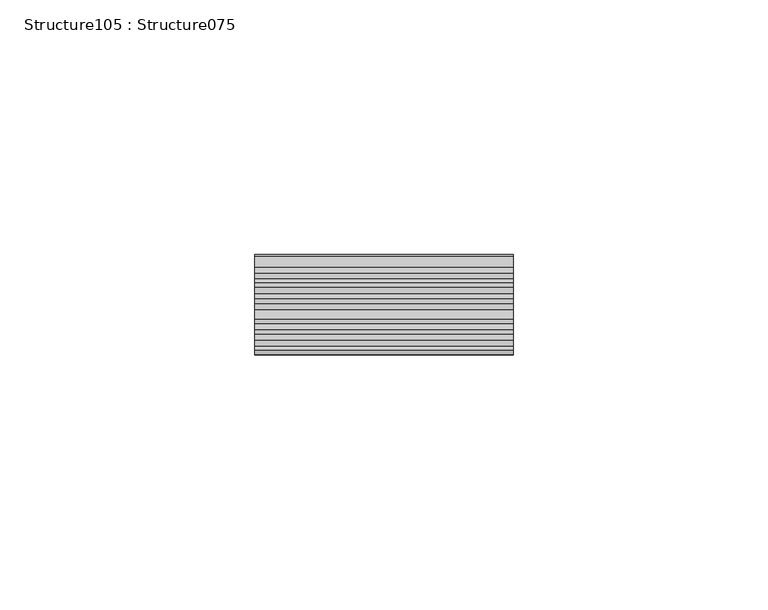
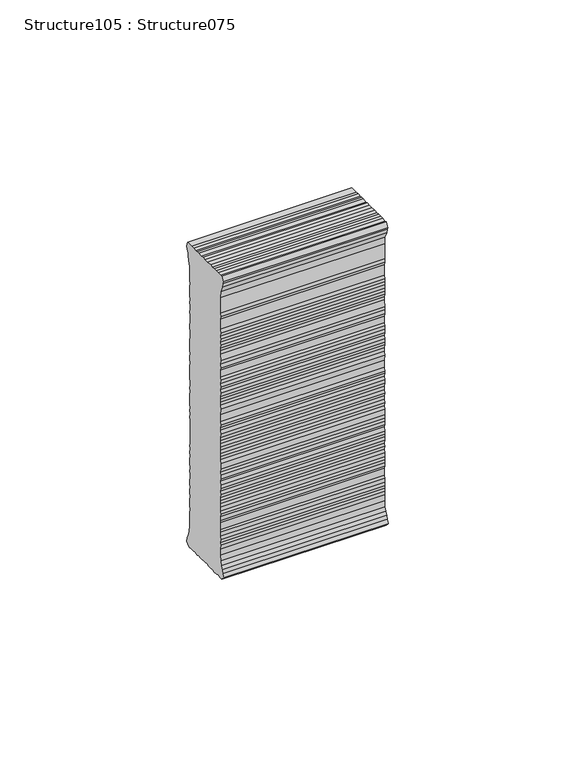
"""IFC4 building model written with IfcOpenShell, lengths in millimetres: proxy geometry, Structure105 : Structure075."""

from ifc_helpers import new_model, si_unit, frame, origin, place, context, project, spatial, polyline, outline, extrude, source, transform, mapped, element, save


def structure105_structure075_dffd82cc(model_context):
    return source(origin(), model_context, "Body", "SweptSolid", [
        extrude(outline(polyline([(1.8233335, 0.0), (3.1470297, 0.293028), (4.2244865, 0.737662), (5.4061289, 0.9114746), (6.4793271, 1.3564168), (7.453505, 0.3744049), (7.3876839, -0.5348157), (7.0413299, -1.6823692), (7.2469213, -2.4792419), (7.1626024, -3.6439812), (6.9587855, -4.6705706), (7.0218141, -5.5887623), (6.8180229, -6.6149967), (6.6191448, -7.5142283), (6.677363, -8.5580034), (6.5082886, -10.8935151), (6.3003415, -11.9180218), (6.5059586, -12.7145395), (6.1595789, -13.8624479), (6.2363462, -14.6499946), (6.1423932, -15.9478166), (6.1963785, -16.9909285), (6.0112391, -17.759515), (5.0532803, -18.342299), (3.7708431, -18.1196038), (2.7725399, -17.5250563), (1.8899032, -17.0723054), (1.0114786, -16.6155787), (-1.0399, -16.2077185), (-2.0754605, -16.1327513), (-3.1246312, -16.1866547), (-5.1943325, -16.036823), (-6.3503054, -15.693427), (-7.5226219, -15.7384156), (-8.43871, -15.8019532), (-9.3454464, -15.736312), (-10.6227907, -15.3841295), (-11.6774093, -15.5674945), (-12.7168735, -15.4922447), (-13.5992284, -15.1686566), (-14.5213496, -15.2317576), (-15.6843145, -15.1475672), (-16.7108781, -14.9433954), (-17.7503424, -14.8681455), (-18.7938349, -14.9224601), (-19.9492226, -14.7089623), (-21.0077449, -14.8920446), (-21.9144813, -14.8264034), (-22.8118661, -14.6315832), (-23.8366554, -14.4275398), (-24.8819223, -14.4817259), (-26.0451176, -14.2676629), (-26.9573019, -14.3314832), (-28.1165932, -14.1177028), (-35.504632, -13.5828614), (-36.2915412, -13.6557508), (-37.5800115, -13.4326187), (-38.6231492, -13.4869589), (-39.3938393, -13.3013105), (-40.5661558, -13.3462991), (-41.4822438, -13.4098367), (-42.5127113, -13.2053823), (-43.6850278, -13.2503708), (-44.8310639, -12.9076942), (-45.7510557, -12.9709493), (-46.904669, -12.7575799), (-47.9441332, -12.6823301), (-48.9987517, -12.8656951), (-50.9453073, -12.7247783), (-51.8391432, -12.5302151), (-53.1348358, -12.4364162), (-54.0325755, -12.2415703), (-55.2105702, -12.2861478), (-56.2447111, -12.2112834), (-57.1420959, -12.0164631), (-58.057829, -12.0800265), (-60.395825, -11.9107723), (-61.434704, -11.9654207), (-62.4561747, -11.6317617), (-64.2753257, -11.5000681), (-65.4479971, -11.545031), (-66.358407, -11.6089797), (-67.514025, -11.2656093), (-69.5837263, -11.1157777), (-70.5095209, -11.3084686), (-71.7865103, -10.9563118), (-72.8220707, -10.8813446), (-73.6093348, -10.9542083), (-74.7633029, -10.7408132), (-75.814248, -10.7945883), (-76.7303361, -10.8581259), (-78.9327652, -10.6986857), (-79.8207983, -10.3746866), (-80.9987931, -10.4192641), (-85.2712784, -10.1099666), (-87.1286228, -10.4960018), (-88.4487235, -10.7935711), (-89.368916, -10.8546711), (-90.3000349, -11.180043), (-91.3524984, -11.3632072), (-92.6260665, -10.8800153), (-92.4666006, -8.6772313), (-92.5113322, -7.501366), (-92.307032, -6.4730278), (-92.3799983, -5.6871834), (-92.3142543, -4.7790274), (-91.9643553, -3.5036582), (-92.1549168, -2.5780178), (-91.950591, -1.5493248), (-91.7392225, -0.393783), (-91.86404, 1.4400135), (-91.5421703, 2.3282008), (-91.7139001, 3.5139734), (-91.5191057, 4.4110033), (-91.5637858, 5.5875785), (-91.2230844, 6.735898), (-91.4229975, 7.5323595), (-89.9359318, 8.2045553), (-89.1900807, 7.7595664), (-87.9038939, 7.5344593), (-85.9090056, 6.3511965), (-83.842777, 6.0696199), (-78.9197837, 5.7132303), (-77.74128, 5.7599113), (-76.8537302, 5.4341636), (-73.4823032, 5.1900963), (-72.4272012, 5.3752099), (-71.4032759, 5.1690886), (-70.4866788, 5.2347299), (-69.3275415, 5.0188203), (-68.4109444, 5.0844615), (-67.3845349, 4.8781604), (-66.4867694, 4.6836695), (-65.4473053, 4.6084197), (-63.3587722, 4.7187202), (-62.199635, 4.5028106), (-61.0268094, 4.5499027), (-60.1335814, 4.2237439), (-57.9364757, 4.0646891), (-57.137957, 4.2683775), (-55.8517702, 4.0432704), (-54.8059941, 4.09956), (-53.9145406, 3.7735296), (-52.8597935, 3.9586689), (-51.7063344, 3.7431704), (-50.799598, 3.6775291), (-49.7726538, 3.4736865), (-48.7331896, 3.3984367), (-47.5457148, 3.5739675), (-45.7507187, 3.1825271), (-43.4191107, 3.0137353), (-42.3664931, 3.1990287), (-41.5959571, 3.011251), (-40.565464, 2.8071516), (-39.5128462, 2.992445), (-38.2305631, 2.7676205), (-37.20007, 2.563521), (-36.1641547, 2.4885281), (-35.1189134, 2.5423592), (-34.0887752, 2.3382854), (-33.0546342, 2.263421), (-32.0058441, 2.3169952), (-30.9792548, 2.1131783), (-29.9245077, 2.2983176), (-28.11068, 2.1670094), (-26.9533171, 1.9512282), (-26.0370749, 2.0168951), (-24.8723356, 1.9325763), (-23.9805271, 1.6065203), (-22.7987305, 1.7824621), (-21.7628152, 1.7074692), (-20.8595515, 1.510083), (-19.8162597, 1.5665524), (-18.6664484, 1.2218188), (-17.750031, 1.2849758), (-16.7234417, 1.081159), (-15.6803297, 1.1351442), (-14.3846372, 1.0413453), (-13.46804, 1.1069865), (-12.4359523, 0.9002744), (-11.2729874, 0.816084), (-10.5047558, 0.6309704), (-8.1727929, 0.4621529), (-7.3837802, 0.5345331), (-6.0880875, 0.4407342), (-5.0426664, 0.4970495), (-4.0123531, 0.2904658), (-3.2288387, 0.3657413), (-1.9426518, 0.1406342), (0.0, 0.0), (1.8233335, 0.0)])), frame((-56111.290314, 291762.6571238, -368.1935385), z_axis=(-0.9999998917542984, 0.0004652863545059616, 0.0), x_axis=(-3.359550091616789e-05, -0.07220391691855116, -0.9973898902901319)), (0.0, 0.0, 1.0), 50.8),
    ])


if __name__ == "__main__":
    model = new_model("IFC4")
    model_context = context("Model", 3, world=origin())
    ifc_project = project(units=[si_unit("LENGTHUNIT", "METRE", prefix="MILLI")], contexts=[model_context])
    site = spatial("IfcSite", under=ifc_project)
    building = spatial("IfcBuilding", under=site)
    placement = place(None, origin())
    structure105_structure075_shape = structure105_structure075_dffd82cc(model_context)
    element("IfcBuildingElementProxy", 1, Name="Structure105 : Structure075", ObjectType="Structure105 : Structure075", at=placement, inside=building, context=model_context, shape_type="MappedRepresentation", body=[
        mapped(structure105_structure075_shape, transform((0.0, 0.0, 0.0), x_axis=(1.0, 0.0, 0.0), y_axis=(0.0, 1.0, 0.0), z_axis=(0.0, 0.0, 1.0))),
    ])
    save(model, "model.ifc")

# Revit data of these elements
# Type "Structure105 : Structure075"
#   NameOverride = "Structure075"
# Element 1 (IfcBuildingElementProxy, "Structure105 : Structure075")
#   Materials on its faces: "BRUSHED ALUMINUM LETTERING"
# Materials
#   "BRUSHED ALUMINUM LETTERING": class "Unassigned", colour RGB 169 181 186, transparency 0, Cost = 0
